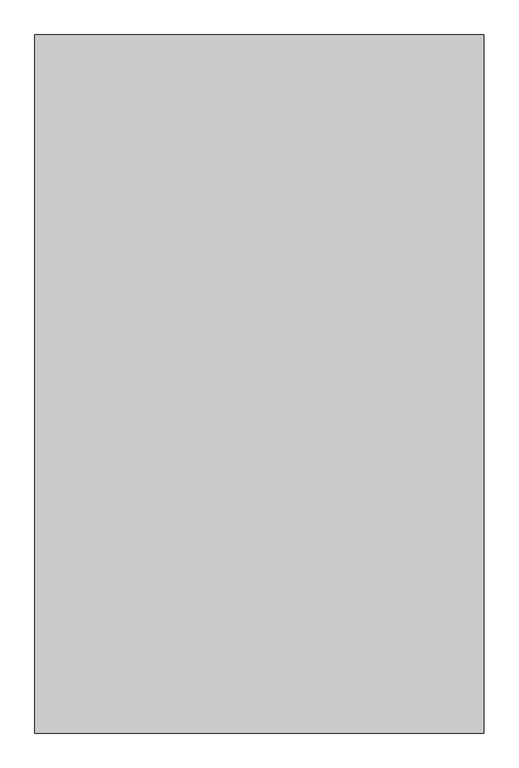
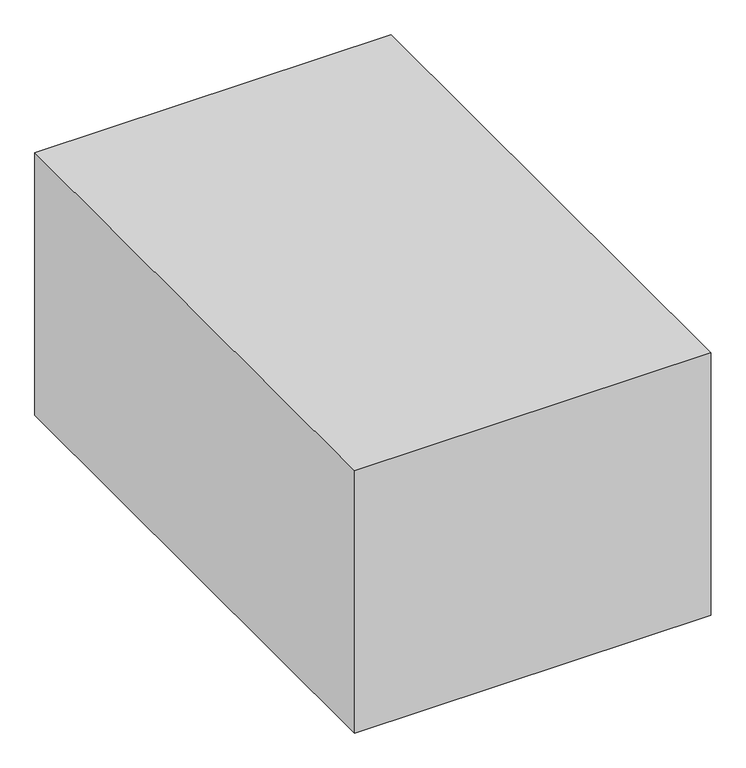
"""IFC4 building model written with IfcOpenShell, lengths in millimetres: proxy geometry, Space Planning Box_hec : Space Planning Box_hec."""

from ifc_helpers import new_model, si_unit, origin, origin_with_axes, place, context, project, spatial, polyline, outline, extrude, source, transform, mapped, element, save


def generic_models_10b6925f(model_context):
    return source(origin(), model_context, "Body", "SweptSolid", [
        extrude(outline(polyline([(2250.0, 3500.0), (2250.0, -3500.0), (-2250.0, -3500.0), (-2250.0, 3500.0), (2250.0, 3500.0)])), origin_with_axes(), (0.0, 0.0, 1.0), 3500.0),
    ])


if __name__ == "__main__":
    model = new_model("IFC4")
    model_context = context("Model", 3, world=origin())
    ifc_project = project(units=[si_unit("LENGTHUNIT", "METRE", prefix="MILLI")], contexts=[model_context])
    site = spatial("IfcSite", under=ifc_project)
    building = spatial("IfcBuilding", under=site)
    placement = place(None, origin())
    generic_models_shape = generic_models_10b6925f(model_context)
    element("IfcBuildingElementProxy", 1, Name="Space Planning Box_hec : Space Planning Box_hec", ObjectType="Space Planning Box_hec : Space Planning Box_hec", at=placement, inside=building, context=model_context, shape_type="MappedRepresentation", body=[
        mapped(generic_models_shape, transform((0.0, 0.0, 0.0), x_axis=(1.0, 0.0, 0.0), y_axis=(0.0, 1.0, 0.0), z_axis=(0.0, 0.0, 1.0))),
    ])
    save(model, "model.ifc")

# Revit data of these elements
# Type "Space Planning Box_hec : Space Planning Box_hec"
#   Type Comments = "..."
#   Room Name [instance default] = "?"
#   Interior Finish [instance default] = ""
#   Exterior Finish [instance default] = ""
#   Department [instance default] = ""
#   Assembly Code = "..."
#   ceiling height [instance default] = 0
#   Width [instance default] = 1524 mm
#   Program Area [instance default] = 0.00 m²
#   Length [instance default] = 1524 mm
#   Height [instance default] = 1524 mm
#   Area [instance default] = 2.32258 m²
#   Fill Color [instance default] = Cyan
#   Default Elevation = 0
# Element 1 (IfcBuildingElementProxy, "Space Planning Box_hec : Space Planning Box_hec")
#   Room Name = "Break Room"
#   Exterior Finish = "RF1..N/A,,EW2..N/A..N/A"
#   Department = "AR"
#   Width = 4500 mm
#   Program Area = 31.50 m²
#   Length = 7000 mm
#   Height = 3500 mm
#   Area = 31.50 m²
#   Materials on its faces: "Cyan"
# Materials
#   "Cyan": class "Generic", colour RGB 0 255 255, transparency 0.2, Cost = 0
